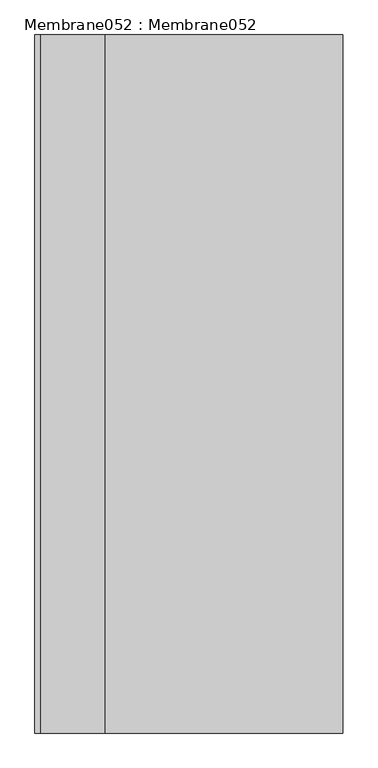
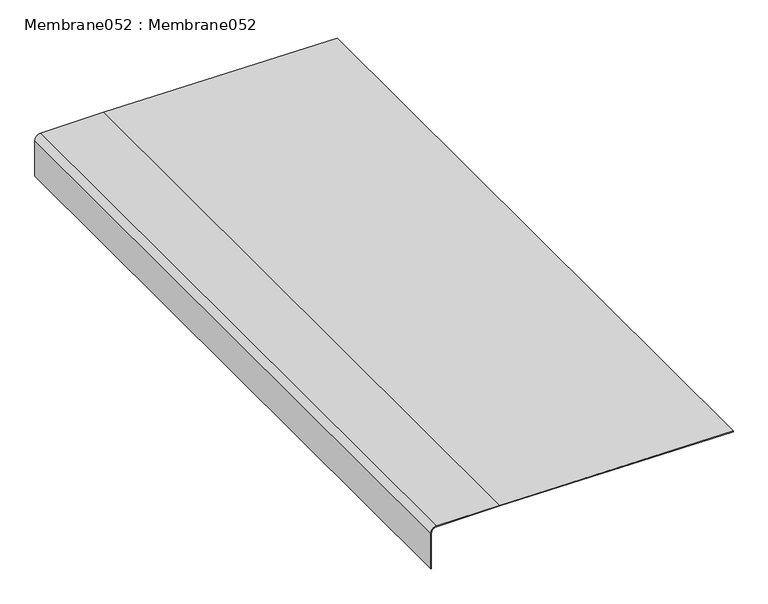
"""IFC4 building model written with IfcOpenShell, lengths in millimetres: proxy geometry, Membrane052 : Membrane052."""

from ifc_helpers import new_model, si_unit, point, frame, frame_2d, origin, place, context, project, spatial, polyline, circle_curve, trimmed, segment, composite_curve, outline, extrude, source, transform, mapped, element, save


def membrane052_membrane052_4266f00a(model_context):
    return source(origin(), model_context, "Body", "SweptSolid", [
        extrude(outline(composite_curve([segment(trimmed(circle_curve(frame_2d((40234.8417335, -2761.2384069)), 15.0), [point((40234.8417335, -2776.2384069))], [point((40249.8417335, -2761.2384069))], True, "CARTESIAN"), True, "CONTINUOUS"), segment(polyline([(40249.8417335, -2761.2384069), (40249.8417335, -2577.3779567), (40240.0438802, -1896.5672037), (40242.0436731, -1896.5384237), (40251.8417335, -2577.3635659), (40251.8417335, -2761.2384069)]), True, "CONTINUOUS"), segment(trimmed(circle_curve(frame_2d((40234.8417335, -2761.2384069)), 17.0), [point((40251.8417335, -2761.2384069))], [point((40234.8417335, -2778.2384069))], False, "CARTESIAN"), True, "CONTINUOUS"), segment(polyline([(40234.8417335, -2778.2384069), (40125.2457074, -2778.2384069), (40125.2457074, -2776.2384069), (40234.8417335, -2776.2384069)]), True, "CONTINUOUS")], self_intersect=False)), frame((0.0, -1052.8906574, 0.0), z_axis=(0.0, 1.0, 0.0), x_axis=(0.0, 0.0, 1.0)), (0.0, 0.0, 1.0), 2000.0),
    ])


if __name__ == "__main__":
    model = new_model("IFC4")
    model_context = context("Model", 3, world=origin())
    ifc_project = project(units=[si_unit("LENGTHUNIT", "METRE", prefix="MILLI")], contexts=[model_context])
    site = spatial("IfcSite", under=ifc_project)
    building = spatial("IfcBuilding", under=site)
    placement = place(None, origin())
    membrane052_membrane052_shape = membrane052_membrane052_4266f00a(model_context)
    element("IfcBuildingElementProxy", 1, Name="Membrane052 : Membrane052", ObjectType="Membrane052 : Membrane052", at=placement, inside=building, context=model_context, shape_type="MappedRepresentation", body=[
        mapped(membrane052_membrane052_shape, transform((0.0, 0.0, 0.0), x_axis=(1.0, 0.0, 0.0), y_axis=(0.0, 1.0, 0.0), z_axis=(0.0, 0.0, 1.0))),
    ])
    save(model, "model.ifc")

# Revit data of these elements
# Type "Membrane052 : Membrane052"
#   NameOverride = "Membrane052"
# Element 1 (IfcBuildingElementProxy, "Membrane052 : Membrane052")
#   Materials on its faces: "THREE PLY BUILT UP ROOF MEMBRANE"
# Materials
#   "THREE PLY BUILT UP ROOF MEMBRANE": class "Unassigned", colour RGB 63 63 63, transparency 0
